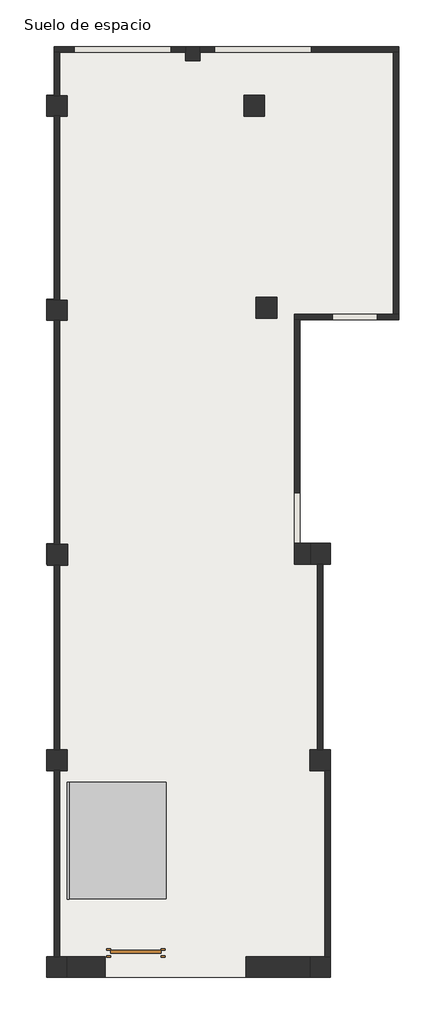
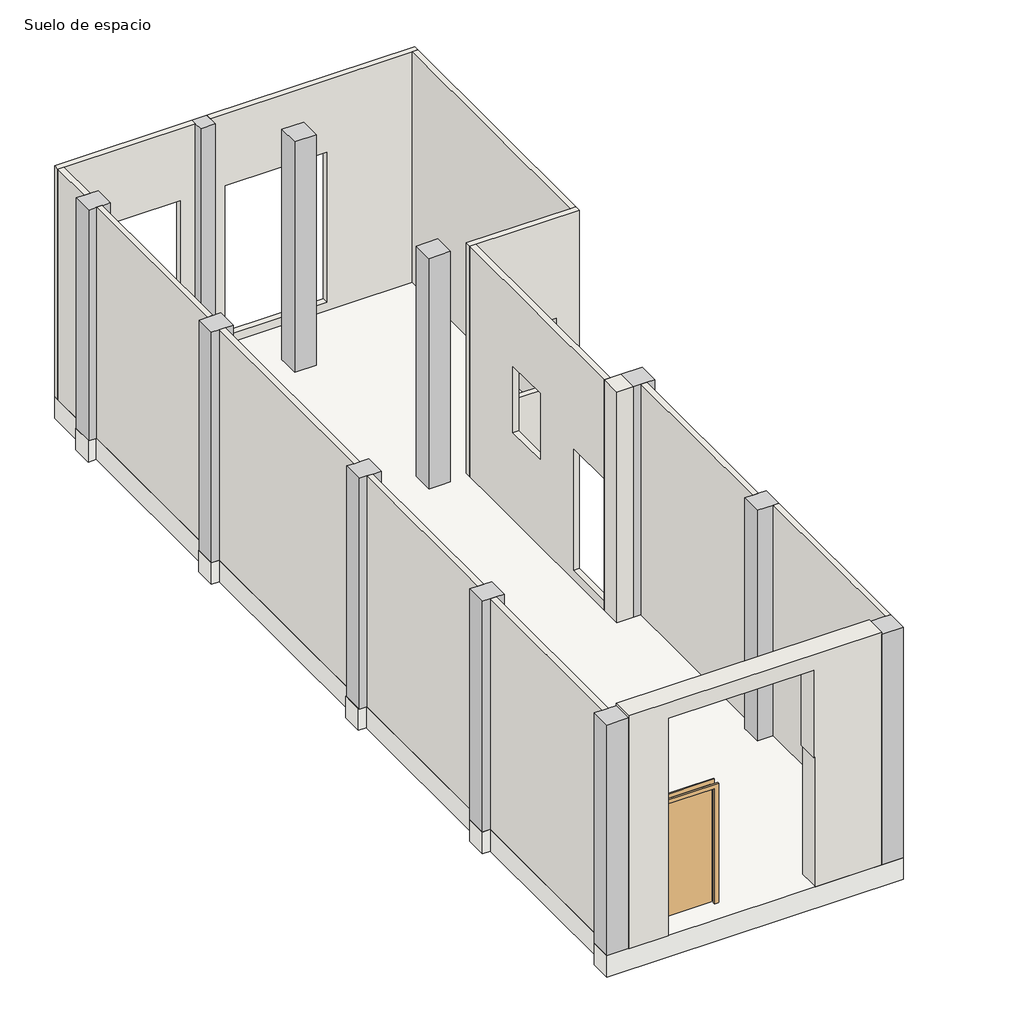
# One storey: 14 walls, 11 columns, 1 door, 1 railing, 1 ramp, 1 slab.
"""IFC4 building model written with IfcOpenShell, lengths in millimetres."""

import ifcopenshell
import ifcopenshell.guid

model = None  # the IFC model being written
_history = None  # IfcOwnerHistory: only IFC2X3 demands one
_inside = {}  # id of a spatial element -> (the spatial element, [elements in it])
_under = {}  # id of a project, library or spatial element -> (it, [spatial elements below it])
_declared = {}  # id of a project -> (the project, [libraries it declares])
_typed = {}  # id of a type object -> (the type object, [elements of that type])
_made_of = {}  # id of a material, layer set ... -> (it, [elements and type objects made of it])


def new_model(schema):
    """Start an empty IFC model of exactly this schema.

    Asked for "IFC4X3", IfcOpenShell would pick the latest addendum, in which some entities
    have other attributes; the version numbers below select the first issue.
    IFC2X3 requires an IfcOwnerHistory on every rooted entity: one is made here for all.
    """
    global model, _history
    if schema == "IFC4X3":
        model = ifcopenshell.file(schema_version=(4, 3, 0, 0))
    else:
        model = ifcopenshell.file(schema=schema)
    _inside.clear()
    _under.clear()
    _declared.clear()
    _typed.clear()
    _made_of.clear()
    _history = None
    if model.schema == "IFC2X3":
        org = make("IfcOrganization", Name="unknown")
        user = make(
            "IfcPersonAndOrganization",
            ThePerson=make("IfcPerson", FamilyName="unknown"),
            TheOrganization=org,
        )
        app = make(
            "IfcApplication",
            ApplicationDeveloper=org,
            Version="unknown",
            ApplicationFullName="unknown",
            ApplicationIdentifier="unknown",
        )
        _history = make(
            "IfcOwnerHistory",
            OwningUser=user,
            OwningApplication=app,
            ChangeAction="ADDED",
            CreationDate=0,
        )
    return model


def make(cls, **values):
    """One entity of the class cls with the attributes given. An attribute that is None is left unset."""
    return model.create_entity(
        cls, **{name: value for name, value in values.items() if value is not None}
    )


def rooted(cls, **values):
    """An entity with a GlobalId (a new one), such as an element, a storey or a relation."""
    return make(cls, GlobalId=ifcopenshell.guid.new(), OwnerHistory=_history, **values)


def si_unit(unit_type, name, prefix=None):
    """IfcSIUnit, for example si_unit("LENGTHUNIT", "METRE", prefix="MILLI")."""
    return make("IfcSIUnit", UnitType=unit_type, Prefix=prefix, Name=name)


def assignment(units):
    """IfcUnitAssignment: the units of a project."""
    return None if units is None else make("IfcUnitAssignment", Units=units)


def point(xyz):
    """IfcCartesianPoint."""
    return None if xyz is None else make("IfcCartesianPoint", Coordinates=xyz)


def direction(xyz):
    """IfcDirection."""
    return None if xyz is None else make("IfcDirection", DirectionRatios=xyz)


def frame(location, z_axis=None, x_axis=None):
    """IfcAxis2Placement3D, a coordinate frame: its origin and axes. An axis left out is left unset."""
    return make(
        "IfcAxis2Placement3D",
        Location=point(location),
        Axis=direction(z_axis),
        RefDirection=direction(x_axis),
    )


def origin():
    """The frame at (0, 0, 0) with its axes left unset."""
    return frame((0.0, 0.0, 0.0))


def origin_with_axes():
    """The frame at (0, 0, 0) with the z axis (0, 0, 1) and the x axis (1, 0, 0) written out."""
    return frame((0.0, 0.0, 0.0), z_axis=(0.0, 0.0, 1.0), x_axis=(1.0, 0.0, 0.0))


def place(relative_to, where):
    """IfcLocalPlacement: puts the frame where relative to a parent placement (None: the world)."""
    return make(
        "IfcLocalPlacement", PlacementRelTo=relative_to, RelativePlacement=where
    )


def context(
    kind, dimensions, precision=None, world=None, true_north=None, identifier=None
):
    """IfcGeometricRepresentationContext, for example the 3D "Model" context."""
    return make(
        "IfcGeometricRepresentationContext",
        ContextIdentifier=identifier,
        ContextType=kind,
        CoordinateSpaceDimension=dimensions,
        Precision=precision,
        WorldCoordinateSystem=world,
        TrueNorth=true_north,
    )


def project(units=None, contexts=None):
    """IfcProject with its units and contexts."""
    return rooted(
        "IfcProject",
        Name="project",
        RepresentationContexts=contexts,
        UnitsInContext=assignment(units),
    )


def spatial(cls, under=None, at=None, **own):
    """A site, building, storey or space (cls), placed at a placement, below another one or the project."""
    s = rooted(cls, ObjectPlacement=at, **own)
    if under is not None:
        _under.setdefault(under.id(), (under, []))[1].append(s)
    return s


def polyline(points):
    """IfcPolyline through the points."""
    return make("IfcPolyline", Points=[point(p) for p in points])


def ellipse_curve(where, semi_axis1, semi_axis2):
    """IfcEllipse in the frame where."""
    return make(
        "IfcEllipse", Position=where, SemiAxis1=semi_axis1, SemiAxis2=semi_axis2
    )


def outline(outer, holes=None, kind="AREA"):
    """IfcArbitraryClosedProfileDef: a profile drawn as a closed curve; with holes, ...WithVoids."""
    if holes is None:
        return make("IfcArbitraryClosedProfileDef", ProfileType=kind, OuterCurve=outer)
    return make(
        "IfcArbitraryProfileDefWithVoids",
        ProfileType=kind,
        OuterCurve=outer,
        InnerCurves=holes,
    )


def extrude(swept, where, along, depth):
    """IfcExtrudedAreaSolid: the profile swept, set in the frame where, extruded along a direction by depth."""
    return make(
        "IfcExtrudedAreaSolid",
        SweptArea=swept,
        Position=where,
        ExtrudedDirection=direction(along),
        Depth=depth,
    )


def faces_of(points, faces, orient=None, outer=None):
    """IfcFace entities. A face is a list of loops; a loop is a list of indices into points, from 0.

    orient and outer hold one flag for each loop. By default every Orientation is true, the
    first loop of a face is its IfcFaceOuterBound and the others are IfcFaceBound.
    """
    made = []
    for i, loops in enumerate(faces):
        bounds = []
        for j, loop in enumerate(loops):
            is_outer = j == 0 if outer is None else outer[i][j]
            bounds.append(
                make(
                    "IfcFaceOuterBound" if is_outer else "IfcFaceBound",
                    Bound=make("IfcPolyLoop", Polygon=[points[k] for k in loop]),
                    Orientation=True if orient is None else orient[i][j],
                )
            )
        made.append(make("IfcFace", Bounds=bounds))
    return made


def faceted_brep(points, faces, orient=None, outer=None, voids=None):
    """IfcFacetedBrep: a solid bounded by flat faces; with voids (closed shells), ...WithVoids."""
    shared = [point(p) for p in points]
    hull = make("IfcClosedShell", CfsFaces=faces_of(shared, faces, orient, outer))
    if voids is None:
        return make("IfcFacetedBrep", Outer=hull)
    return make(
        "IfcFacetedBrepWithVoids",
        Outer=hull,
        Voids=[
            make(cls, CfsFaces=faces_of(shared, fs, o, b)) for cls, fs, o, b in voids
        ],
    )


def shape(context_of_items, identifier, shape_type, items):
    """IfcShapeRepresentation: the items that make up one representation, for example the "Body"."""
    return make(
        "IfcShapeRepresentation",
        ContextOfItems=context_of_items,
        RepresentationIdentifier=identifier,
        RepresentationType=shape_type,
        Items=items,
    )


def source(mapping_origin, context_of_items, identifier, shape_type, items):
    """IfcRepresentationMap: a shape defined once, which mapped items show again and again."""
    return make(
        "IfcRepresentationMap",
        MappingOrigin=mapping_origin,
        MappedRepresentation=shape(context_of_items, identifier, shape_type, items),
    )


def transform(
    local_origin,
    x_axis=None,
    y_axis=None,
    z_axis=None,
    scale=None,
    scale2=None,
    scale3=None,
    uniform=True,
):
    """IfcCartesianTransformationOperator3D, or its non-uniform kind. x_axis, y_axis, z_axis: its Axis1, 2, 3."""
    if uniform:
        return make(
            "IfcCartesianTransformationOperator3D",
            Axis1=direction(x_axis),
            Axis2=direction(y_axis),
            LocalOrigin=point(local_origin),
            Scale=scale,
            Axis3=direction(z_axis),
        )
    return make(
        "IfcCartesianTransformationOperator3DnonUniform",
        Axis1=direction(x_axis),
        Axis2=direction(y_axis),
        LocalOrigin=point(local_origin),
        Scale=scale,
        Axis3=direction(z_axis),
        Scale2=scale2,
        Scale3=scale3,
    )


def mapped(mapping_source, mapping_target):
    """IfcMappedItem: shows the shape of a source again, moved by a transform."""
    return make(
        "IfcMappedItem", MappingSource=mapping_source, MappingTarget=mapping_target
    )


def made_of(thing, what):
    """Note that an element or type object is made of a material, layer set ...; save() writes the relation."""
    if what is not None:
        _made_of.setdefault(what.id(), (what, []))[1].append(thing)
    return thing


def element(
    cls,
    number,
    at=None,
    inside=None,
    cuts=None,
    type_object=None,
    material=None,
    context=None,
    identifier="Body",
    shape_type=None,
    held_by="IfcProductDefinitionShape",
    body=None,
    shapes=None,
    **own,
):
    """One element of the class cls, such as IfcWall. Its Tag is "e" and its number.

    at: its placement. inside: the storey or other place that contains it. cuts: it is an
    opening in that element (IfcRelVoidsElement). A single representation is given by context,
    identifier, shape_type and body (its items); several are given by shapes. held_by: the class
    of the entity that holds the representations. save() writes the other relations.
    """
    e = rooted(cls, Tag="e%d" % number, ObjectPlacement=at, **own)
    if body is not None:
        shapes = [shape(context, identifier, shape_type, body)]
    if shapes is not None:
        e.Representation = make(held_by, Representations=shapes)
    if inside is not None:
        _inside.setdefault(inside.id(), (inside, []))[1].append(e)
    if cuts is not None:
        rooted(
            "IfcRelVoidsElement", RelatingBuildingElement=cuts, RelatedOpeningElement=e
        )
    if type_object is not None:
        _typed.setdefault(type_object.id(), (type_object, []))[1].append(e)
    return made_of(e, material)


def aggregate(whole, parts):
    """IfcRelAggregates: a whole, such as a stair, and the parts it consists of."""
    return rooted("IfcRelAggregates", RelatingObject=whole, RelatedObjects=parts)


def save(model, path):
    """Write the relations noted so far, then the file.

    IfcRelAggregates (storeys below a building ...), IfcRelContainedInSpatialStructure (elements
    in a storey), IfcRelDefinesByType, IfcRelAssociatesMaterial and IfcRelDeclares: one each for
    every whole, place, type object, material and project.
    """
    for whole, parts in _under.values():
        aggregate(whole, parts)
    for where, things in _inside.values():
        rooted(
            "IfcRelContainedInSpatialStructure",
            RelatedElements=things,
            RelatingStructure=where,
        )
    for kind, things in _typed.values():
        rooted("IfcRelDefinesByType", RelatedObjects=things, RelatingType=kind)
    for what, things in _made_of.values():
        rooted("IfcRelAssociatesMaterial", RelatedObjects=things, RelatingMaterial=what)
    for by, libraries in _declared.values():
        rooted("IfcRelDeclares", RelatingContext=by, RelatedDefinitions=libraries)
    model.write(path)


def plane_surface(at):
    """IfcPlane: the flat surface through the origin of the frame at, square to its z axis."""
    return make("IfcPlane", Position=at)


def cylinder_surface(at, radius):
    """IfcCylindricalSurface: all points at the distance radius from the z axis of the frame at."""
    return make("IfcCylindricalSurface", Position=at, Radius=radius)


def advanced_brep(points, edges, surfaces, faces):
    """IfcAdvancedBrep: a solid bounded by faces that lie on surfaces and meet in shared edges.

    An edge is (start, end): straight between two places in points (the first is 0);
    or (start, end, curve); or (start, end, curve, False) where it runs against its curve.
    A face is (place in surfaces, loops), or (place, loops, False) where it looks against
    its surface's normal. A loop lists edges by number (the first is 1), with a minus sign
    where the edge is run from its end to its start. The first loop is the outer one.
    """
    corners = [point(p) for p in points]
    vertices = [make("IfcVertexPoint", VertexGeometry=c) for c in corners]
    made = []
    for start, end, *more in edges:
        made.append(
            make(
                "IfcEdgeCurve",
                EdgeStart=vertices[start],
                EdgeEnd=vertices[end],
                EdgeGeometry=more[0] if more else make("IfcPolyline", Points=[corners[start], corners[end]]),
                SameSense=more[1] if len(more) > 1 else True,
            )
        )
    hull = []
    for where, loops, *sense in faces:
        bounds = []
        for j, loop in enumerate(loops):
            ring = [make("IfcOrientedEdge", EdgeElement=made[abs(k) - 1], Orientation=k > 0) for k in loop]
            bounds.append(
                make(
                    "IfcFaceOuterBound" if j == 0 else "IfcFaceBound",
                    Bound=make("IfcEdgeLoop", EdgeList=ring),
                    Orientation=True,
                )
            )
        hull.append(make("IfcAdvancedFace", Bounds=bounds, FaceSurface=surfaces[where], SameSense=sense[0] if sense else True))
    return make("IfcAdvancedBrep", Outer=make("IfcClosedShell", CfsFaces=hull))


def m_rectangular_column_380_x_380mm_f7aa0fc7(model_context):
    return source(origin(), model_context, "Body", "SweptSolid", [
        extrude(outline(polyline([(190.0, 190.0), (190.0, -190.0), (-190.0, -190.0), (-190.0, 190.0), (190.0, 190.0)])), frame((0.0, 0.0, 40.0), z_axis=(0.0, 0.0, 1.0), x_axis=(1.0, 0.0, 0.0)), (0.0, 0.0, 1.0), 4260.0),
    ])


def m_single_flush_0915_x_2134mm_17617764(model_context):
    return source(origin(), model_context, "Body", "SweptSolid", [
        extrude(outline(polyline([(2210.0, -533.5), (0.0, -533.5), (0.0, -457.5), (2134.0, -457.5), (2134.0, 457.5), (0.0, 457.5), (0.0, 533.5), (2210.0, 533.5), (2210.0, -533.5)])), frame((0.0, -75.0, 0.0), z_axis=(0.0, 1.0, 0.0), x_axis=(0.0, 0.0, 1.0)), (0.0, 0.0, 1.0), 25.0),
        extrude(outline(polyline([(2210.0, 533.5), (2210.0, -533.5), (0.0, -533.5), (0.0, -457.5), (2134.0, -457.5), (2134.0, 457.5), (0.0, 457.5), (0.0, 533.5), (2210.0, 533.5)])), frame((0.0, 50.0, 0.0), z_axis=(0.0, 1.0, 0.0), x_axis=(0.0, 0.0, 1.0)), (0.0, 0.0, 1.0), 25.0),
        extrude(outline(polyline([(457.5, 1.0), (457.5, -50.0), (-457.5, -50.0), (-457.5, 1.0), (457.5, 1.0)])), origin_with_axes(), (0.0, 0.0, 1.0), 2134.0),
    ])


def ramp_1_b614bedc(model_context):
    return source(origin(), model_context, "Body", "SweptSolid", [
        extrude(outline(polyline([(-588.7354398, 40.0), (1550.939444, 200.0), (1550.939444, 49.5812066), (-588.7354398, -110.4187934), (-588.7354398, 40.0)])), frame((5737.3508412, 0.0, 0.0), z_axis=(1.0, 0.0, 0.0), x_axis=(0.0, 1.0, 0.0)), (0.0, 0.0, 1.0), 1790.0),
    ])


model = new_model("IFC4")

# Units and contexts
model_context = context("Model", 3, world=origin())
ifc_project = project(units=[si_unit("LENGTHUNIT", "METRE", prefix="MILLI")], contexts=[model_context])

# Site, building, storey
site = spatial("IfcSite", under=ifc_project)
building = spatial("IfcBuilding", under=site)
storey = spatial("IfcBuildingStorey", under=building, Name="Suelo de espacio", Elevation=40.0)

# Columns
placement = place(None, origin())
element("IfcColumn", 1, ObjectType="M_Rectangular Column : 260 x 260mm", at=placement, inside=storey, context=model_context, shape_type="Brep", body=[
    faceted_brep([(8142.3508412, 14950.939444, 4300.0), (7882.3508412, 14950.939444, 4300.0), (7882.3508412, 14850.939444, 4300.0), (7882.3508412, 14690.939444, 4300.0), (8142.3508412, 14690.939444, 4300.0), (8142.3508412, 14850.939444, 4300.0), (8142.3508412, 14950.939444, 40.0), (8142.3508412, 14850.939444, 40.0), (8142.3508412, 14690.939444, 40.0), (7882.3508412, 14690.939444, 40.0), (7882.3508412, 14850.939444, 40.0), (7882.3508412, 14950.939444, 40.0)], [[[0, 1, 2, 3, 4, 5]], [[6, 7, 8, 9, 10, 11]], [[1, 0, 6, 11]], [[3, 2, 1, 11, 10, 9]], [[4, 3, 9, 8]], [[0, 5, 4, 8, 7, 6]]]),
])
element("IfcColumn", 2, ObjectType="M_Rectangular Column : 380 x 370mm", at=placement, inside=storey, context=model_context, shape_type="Brep", body=[
    faceted_brep([(5722.3508412, 10330.939444, 4300.0), (5342.3508412, 10330.939444, 4300.0), (5342.3508412, 9960.939444, 4300.0), (5482.3508412, 9960.939444, 4300.0), (5582.3508412, 9960.939444, 4300.0), (5722.3508412, 9960.939444, 4300.0), (5722.3508412, 10330.939444, 40.0), (5722.3508412, 9960.939444, 40.0), (5582.3508412, 9960.939444, 40.0), (5482.3508412, 9960.939444, 40.0), (5342.3508412, 9960.939444, 40.0), (5342.3508412, 10330.939444, 40.0)], [[[0, 1, 2, 3, 4, 5]], [[6, 7, 8, 9, 10, 11]], [[1, 0, 6, 11]], [[2, 1, 11, 10]], [[5, 4, 3, 2, 10, 9, 8, 7]], [[0, 5, 7, 6]]]),
])
element("IfcColumn", 3, ObjectType="M_Rectangular Column : 380 x 370mm", at=placement, inside=storey, context=model_context, shape_type="Brep", body=[
    faceted_brep([(5722.3508412, 14050.939444, 4300.0), (5582.3508412, 14050.939444, 4300.0), (5482.3508412, 14050.939444, 4300.0), (5342.3508412, 14050.939444, 4300.0), (5342.3508412, 13680.939444, 4300.0), (5482.3508412, 13680.939444, 4300.0), (5482.3508412, 13685.939444, 4300.0), (5582.3508412, 13685.939444, 4300.0), (5582.3508412, 13680.939444, 4300.0), (5722.3508412, 13680.939444, 4300.0), (5722.3508412, 14050.939444, 40.0), (5722.3508412, 13680.939444, 40.0), (5582.3508412, 13680.939444, 40.0), (5582.3508412, 13685.939444, 40.0), (5482.3508412, 13685.939444, 40.0), (5482.3508412, 13680.939444, 40.0), (5342.3508412, 13680.939444, 40.0), (5342.3508412, 14050.939444, 40.0), (5482.3508412, 14050.939444, 40.0), (5582.3508412, 14050.939444, 40.0)], [[[0, 1, 2, 3, 4, 5, 6, 7, 8, 9]], [[10, 11, 12, 13, 14, 15, 16, 17, 18, 19]], [[3, 2, 1, 0, 10, 19, 18, 17]], [[4, 3, 17, 16]], [[4, 16, 15, 5]], [[0, 9, 11, 10]], [[7, 13, 12, 8]], [[14, 6, 5, 15]], [[13, 7, 6, 14]], [[11, 9, 8, 12]]]),
])
element("IfcColumn", 4, ObjectType="M_Rectangular Column : 380 x 380mm", at=placement, inside=storey, context=model_context, shape_type="Brep", body=[
    faceted_brep([(5722.3508412, -1629.060556, 4300.0), (5582.3508412, -1629.060556, 4300.0), (5482.3508412, -1629.060556, 4300.0), (5342.3508412, -1629.060556, 4300.0), (5342.3508412, -2009.060556, 4300.0), (5722.3508412, -2009.060556, 4300.0), (5722.3508412, -1629.060556, 40.0), (5722.3508412, -2009.060556, 40.0), (5342.3508412, -2009.060556, 40.0), (5342.3508412, -1629.060556, 40.0), (5482.3508412, -1629.060556, 40.0), (5582.3508412, -1629.060556, 40.0)], [[[0, 1, 2, 3, 4, 5]], [[6, 7, 8, 9, 10, 11]], [[3, 2, 1, 0, 6, 11, 10, 9]], [[4, 3, 9, 8]], [[5, 4, 8, 7]], [[0, 5, 7, 6]]]),
])
element("IfcColumn", 5, ObjectType="M_Rectangular Column : 380 x 380mm", at=placement, inside=storey, context=model_context, shape_type="Brep", body=[
    faceted_brep([(10522.3508412, -1629.060556, 4300.0), (10422.3508412, -1629.060556, 4300.0), (10142.3508412, -1629.060556, 4300.0), (10142.3508412, -2009.060556, 4300.0), (10522.3508412, -2009.060556, 4300.0), (10522.3508412, -1629.060556, 40.0), (10522.3508412, -2009.060556, 40.0), (10142.3508412, -2009.060556, 40.0), (10142.3508412, -1629.060556, 40.0), (10422.3508412, -1629.060556, 40.0)], [[[0, 1, 2, 3, 4]], [[5, 6, 7, 8, 9]], [[2, 1, 0, 5, 9, 8]], [[3, 2, 8, 7]], [[4, 3, 7, 6]], [[0, 4, 6, 5]]]),
])
element("IfcColumn", 6, ObjectType="M_Rectangular Column : 380 x 380mm", at=placement, inside=storey, context=model_context, shape_type="Brep", body=[
    faceted_brep([(5722.3508412, 2140.939444, 4300.0), (5582.3508412, 2140.939444, 4300.0), (5482.3508412, 2140.939444, 4300.0), (5342.3508412, 2140.939444, 4300.0), (5342.3508412, 1760.939444, 4300.0), (5482.3508412, 1760.939444, 4300.0), (5482.3508412, 1761.3849652, 4300.0), (5582.3508412, 1761.3849652, 4300.0), (5582.3508412, 1760.939444, 4300.0), (5722.3508412, 1760.939444, 4300.0), (5722.3508412, 2140.939444, 40.0), (5722.3508412, 1760.939444, 40.0), (5582.3508412, 1760.939444, 40.0), (5582.3508412, 1761.3849652, 40.0), (5482.3508412, 1761.3849652, 40.0), (5482.3508412, 1760.939444, 40.0), (5342.3508412, 1760.939444, 40.0), (5342.3508412, 2140.939444, 40.0), (5482.3508412, 2140.939444, 40.0), (5582.3508412, 2140.939444, 40.0)], [[[0, 1, 2, 3, 4, 5, 6, 7, 8, 9]], [[10, 11, 12, 13, 14, 15, 16, 17, 18, 19]], [[3, 2, 1, 0, 10, 19, 18, 17]], [[4, 3, 17, 16]], [[4, 16, 15, 5]], [[0, 9, 11, 10]], [[7, 13, 12, 8]], [[14, 6, 5, 15]], [[11, 9, 8, 12]], [[13, 7, 6, 14]]]),
])
element("IfcColumn", 7, ObjectType="M_Rectangular Column : 380 x 380mm", at=placement, inside=storey, context=model_context, shape_type="Brep", body=[
    faceted_brep([(10522.3508412, 2140.939444, 4300.0), (10382.3508412, 2140.939444, 4300.0), (10282.3508412, 2140.939444, 4300.0), (10142.3508412, 2140.939444, 4300.0), (10142.3508412, 1760.939444, 4300.0), (10422.3508412, 1760.939444, 4300.0), (10522.3508412, 1760.939444, 4300.0), (10522.3508412, 2140.939444, 40.0), (10522.3508412, 1760.939444, 40.0), (10422.3508412, 1760.939444, 40.0), (10142.3508412, 1760.939444, 40.0), (10142.3508412, 2140.939444, 40.0), (10282.3508412, 2140.939444, 40.0), (10382.3508412, 2140.939444, 40.0)], [[[0, 1, 2, 3, 4, 5, 6]], [[7, 8, 9, 10, 11, 12, 13]], [[3, 2, 1, 0, 7, 13, 12, 11]], [[4, 3, 11, 10]], [[6, 5, 4, 10, 9, 8]], [[0, 6, 8, 7]]]),
])
element("IfcColumn", 8, ObjectType="M_Rectangular Column : 380 x 380mm", at=placement, inside=storey, context=model_context, shape_type="Brep", body=[
    faceted_brep([(5732.3508412, 5880.939444, 4300.0), (5582.3508412, 5880.939444, 4300.0), (5482.3508412, 5880.939444, 4300.0), (5352.3508412, 5880.939444, 4300.0), (5352.3508412, 5500.939444, 4300.0), (5482.3508412, 5500.939444, 4300.0), (5582.3508412, 5500.939444, 4300.0), (5732.3508412, 5500.939444, 4300.0), (5732.3508412, 5880.939444, 40.0), (5732.3508412, 5500.939444, 40.0), (5582.3508412, 5500.939444, 40.0), (5482.3508412, 5500.939444, 40.0), (5352.3508412, 5500.939444, 40.0), (5352.3508412, 5880.939444, 40.0), (5482.3508412, 5880.939444, 40.0), (5582.3508412, 5880.939444, 40.0)], [[[0, 1, 2, 3, 4, 5, 6, 7]], [[8, 9, 10, 11, 12, 13, 14, 15]], [[3, 2, 1, 0, 8, 15, 14, 13]], [[4, 3, 13, 12]], [[7, 6, 5, 4, 12, 11, 10, 9]], [[0, 7, 9, 8]]]),
])
element("IfcColumn", 9, ObjectType="M_Rectangular Column : 380 x 380mm", at=placement, inside=storey, context=model_context, shape_type="Brep", body=[
    faceted_brep([(10522.3508412, 5520.939444, 4300.0), (10522.3508412, 5900.939444, 4300.0), (10152.3508412, 5900.939444, 4300.0), (10152.3508412, 5520.939444, 4300.0), (10282.3508412, 5520.939444, 4300.0), (10382.3508412, 5520.939444, 4300.0), (10522.3508412, 5900.939444, 40.0), (10522.3508412, 5520.939444, 40.0), (10382.3508412, 5520.939444, 40.0), (10282.3508412, 5520.939444, 40.0), (10152.3508412, 5520.939444, 40.0), (10152.3508412, 5900.939444, 40.0)], [[[0, 1, 2, 3, 4, 5]], [[6, 7, 8, 9, 10, 11]], [[1, 6, 11, 2]], [[7, 0, 5, 4, 3, 10, 9, 8]], [[1, 0, 7, 6]], [[3, 2, 11, 10]]]),
])
m_rectangular_column_380_x_380mm_shape = m_rectangular_column_380_x_380mm_f7aa0fc7(model_context)
element("IfcColumn", 10, ObjectType="M_Rectangular Column : 380 x 380mm", at=placement, inside=storey, context=model_context, shape_type="MappedRepresentation", body=[
    mapped(m_rectangular_column_380_x_380mm_shape, transform((9132.3508412, 13870.939444, 0.0), x_axis=(1.0, 0.0, 0.0), y_axis=(0.0, 1.0, 0.0), z_axis=(0.0, 0.0, 1.0))),
])
element("IfcColumn", 11, ObjectType="M_Rectangular Column : 380 x 380mm", at=placement, inside=storey, context=model_context, shape_type="MappedRepresentation", body=[
    mapped(m_rectangular_column_380_x_380mm_shape, transform((9352.3508412, 10190.939444, 0.0), x_axis=(1.0, 0.0, 0.0), y_axis=(0.0, 1.0, 0.0), z_axis=(0.0, 0.0, 1.0))),
])

# Door
m_single_flush_0915_x_2134mm_shape = m_single_flush_0915_x_2134mm_17617764(model_context)
element("IfcDoor", 12, ObjectType="M_Single-Flush : 0915 x 2134mm", at=placement, inside=storey, context=model_context, shape_type="MappedRepresentation", body=[
    mapped(m_single_flush_0915_x_2134mm_shape, transform((6972.3508412, -1564.060556, 40.0), x_axis=(-1.0, 0.0, 0.0), y_axis=(0.0, -1.0, 0.0), z_axis=(0.0, 0.0, 1.0))),
])

# Railing
element("IfcRailing", 13, ObjectType="900mm Pipe", at=placement, inside=storey, context=model_context, shape_type="AdvancedBrep", body=[
    advanced_brep(
    [(5757.3508412, -588.7354398, 919.9441609), (5717.3508412, -588.7354398, 919.9441609), (5757.3508412, 1550.939444, 1079.9441609), (5717.3508412, 1550.939444, 1079.9441609)],
    [
        (0, 1, ellipse_curve(frame((5737.3508412, -588.7354398, 919.9441609), z_axis=(0.0, -1.0, 0.0), x_axis=(0.0, 0.0, -1.0)), 20.0558391, 20.0)),
        (1, 0, ellipse_curve(frame((5737.3508412, -588.7354398, 919.9441609), z_axis=(0.0, -1.0, 0.0), x_axis=(0.0, 0.0, -1.0)), 20.0558391, 20.0)),
        (2, 3, ellipse_curve(frame((5737.3508412, 1550.939444, 1079.9441609), z_axis=(0.0, 1.0, 0.0), x_axis=(0.0, 0.0, -1.0)), 20.0558391, 20.0)),
        (3, 2, ellipse_curve(frame((5737.3508412, 1550.939444, 1079.9441609), z_axis=(0.0, 1.0, 0.0), x_axis=(0.0, 0.0, -1.0)), 20.0558391, 20.0)),
        (0, 2),
        (3, 1),
    ],
    [
        plane_surface(frame((5737.3508412, -588.7354398, 940.0), z_axis=(0.0, -1.0, 0.0), x_axis=(0.0, 0.0, 1.0))),
        plane_surface(frame((5737.3508412, 1550.939444, 1100.0), z_axis=(0.0, 1.0, 0.0), x_axis=(0.0, 0.0, 1.0))),
        cylinder_surface(frame((5737.3508412, -587.2440494, 920.0556837), z_axis=(0.0, -0.9972158174462339, -0.07456952081809044), x_axis=(-1.0, 0.0, 0.0)), 20.0),
    ],
    [
        (0, [[1, 2]]),
        (1, [[3, 4]]),
        (2, [[-1, 5, -4, 6]]),
        (2, [[-2, -6, -3, -5]]),
    ],
),
    advanced_brep(
    [(5722.3508412, -588.7354398, 799.9581207), (5752.3508412, -588.7354398, 799.9581207), (5722.3508412, 1550.939444, 959.9581207), (5752.3508412, 1550.939444, 959.9581207)],
    [
        (0, 1, ellipse_curve(frame((5737.3508412, -588.7354398, 799.9581207), z_axis=(0.0, -1.0, 0.0), x_axis=(0.0, 0.0, -1.0)), 15.0418793, 15.0)),
        (1, 0, ellipse_curve(frame((5737.3508412, -588.7354398, 799.9581207), z_axis=(0.0, -1.0, 0.0), x_axis=(0.0, 0.0, -1.0)), 15.0418793, 15.0)),
        (2, 3, ellipse_curve(frame((5737.3508412, 1550.939444, 959.9581207), z_axis=(0.0, 1.0, 0.0), x_axis=(0.0, 0.0, -1.0)), 15.0418793, 15.0)),
        (3, 2, ellipse_curve(frame((5737.3508412, 1550.939444, 959.9581207), z_axis=(0.0, 1.0, 0.0), x_axis=(0.0, 0.0, -1.0)), 15.0418793, 15.0)),
        (0, 2),
        (3, 1),
    ],
    [
        plane_surface(frame((5737.3508412, -588.7354398, 815.0), z_axis=(0.0, -1.0, 0.0), x_axis=(0.0, 0.0, 1.0))),
        plane_surface(frame((5737.3508412, 1550.939444, 975.0), z_axis=(0.0, 1.0, 0.0), x_axis=(0.0, 0.0, 1.0))),
        cylinder_surface(frame((5737.3508412, -587.616897, 800.0417627), z_axis=(0.0, -0.9972158174462339, -0.07456952081809044), x_axis=(1.0, 0.0, 0.0)), 15.0),
    ],
    [
        (0, [[1, 2]]),
        (1, [[3, 4]]),
        (2, [[-1, 5, -4, 6]]),
        (2, [[-2, -6, -3, -5]]),
    ],
),
    advanced_brep(
    [(5722.3508412, -588.7354398, 674.9581207), (5752.3508412, -588.7354398, 674.9581207), (5722.3508412, 1550.939444, 834.9581207), (5752.3508412, 1550.939444, 834.9581207)],
    [
        (0, 1, ellipse_curve(frame((5737.3508412, -588.7354398, 674.9581207), z_axis=(0.0, -1.0, 0.0), x_axis=(0.0, 0.0, -1.0)), 15.0418793, 15.0)),
        (1, 0, ellipse_curve(frame((5737.3508412, -588.7354398, 674.9581207), z_axis=(0.0, -1.0, 0.0), x_axis=(0.0, 0.0, -1.0)), 15.0418793, 15.0)),
        (2, 3, ellipse_curve(frame((5737.3508412, 1550.939444, 834.9581207), z_axis=(0.0, 1.0, 0.0), x_axis=(0.0, 0.0, -1.0)), 15.0418793, 15.0)),
        (3, 2, ellipse_curve(frame((5737.3508412, 1550.939444, 834.9581207), z_axis=(0.0, 1.0, 0.0), x_axis=(0.0, 0.0, -1.0)), 15.0418793, 15.0)),
        (0, 2),
        (3, 1),
    ],
    [
        plane_surface(frame((5737.3508412, -588.7354398, 690.0), z_axis=(0.0, -1.0, 0.0), x_axis=(0.0, 0.0, 1.0))),
        plane_surface(frame((5737.3508412, 1550.939444, 850.0), z_axis=(0.0, 1.0, 0.0), x_axis=(0.0, 0.0, 1.0))),
        cylinder_surface(frame((5737.3508412, -587.616897, 675.0417627), z_axis=(0.0, -0.9972158174462339, -0.07456952081809044), x_axis=(1.0, 0.0, 0.0)), 15.0),
    ],
    [
        (0, [[1, 2]]),
        (1, [[3, 4]]),
        (2, [[-1, 5, -4, 6]]),
        (2, [[-2, -6, -3, -5]]),
    ],
),
    advanced_brep(
    [(5722.3508412, -588.7354398, 549.9581207), (5752.3508412, -588.7354398, 549.9581207), (5722.3508412, 1550.939444, 709.9581207), (5752.3508412, 1550.939444, 709.9581207)],
    [
        (0, 1, ellipse_curve(frame((5737.3508412, -588.7354398, 549.9581207), z_axis=(0.0, -1.0, 0.0), x_axis=(0.0, 0.0, -1.0)), 15.0418793, 15.0)),
        (1, 0, ellipse_curve(frame((5737.3508412, -588.7354398, 549.9581207), z_axis=(0.0, -1.0, 0.0), x_axis=(0.0, 0.0, -1.0)), 15.0418793, 15.0)),
        (2, 3, ellipse_curve(frame((5737.3508412, 1550.939444, 709.9581207), z_axis=(0.0, 1.0, 0.0), x_axis=(0.0, 0.0, -1.0)), 15.0418793, 15.0)),
        (3, 2, ellipse_curve(frame((5737.3508412, 1550.939444, 709.9581207), z_axis=(0.0, 1.0, 0.0), x_axis=(0.0, 0.0, -1.0)), 15.0418793, 15.0)),
        (0, 2),
        (3, 1),
    ],
    [
        plane_surface(frame((5737.3508412, -588.7354398, 565.0), z_axis=(0.0, -1.0, 0.0), x_axis=(0.0, 0.0, 1.0))),
        plane_surface(frame((5737.3508412, 1550.939444, 725.0), z_axis=(0.0, 1.0, 0.0), x_axis=(0.0, 0.0, 1.0))),
        cylinder_surface(frame((5737.3508412, -587.616897, 550.0417627), z_axis=(0.0, -0.9972158174462339, -0.07456952081809044), x_axis=(1.0, 0.0, 0.0)), 15.0),
    ],
    [
        (0, [[1, 2]]),
        (1, [[3, 4]]),
        (2, [[-1, 5, -4, 6]]),
        (2, [[-2, -6, -3, -5]]),
    ],
),
    advanced_brep(
    [(5722.3508412, -588.7354398, 424.9581207), (5752.3508412, -588.7354398, 424.9581207), (5722.3508412, 1550.939444, 584.9581207), (5752.3508412, 1550.939444, 584.9581207)],
    [
        (0, 1, ellipse_curve(frame((5737.3508412, -588.7354398, 424.9581207), z_axis=(0.0, -1.0, 0.0), x_axis=(0.0, 0.0, -1.0)), 15.0418793, 15.0)),
        (1, 0, ellipse_curve(frame((5737.3508412, -588.7354398, 424.9581207), z_axis=(0.0, -1.0, 0.0), x_axis=(0.0, 0.0, -1.0)), 15.0418793, 15.0)),
        (2, 3, ellipse_curve(frame((5737.3508412, 1550.939444, 584.9581207), z_axis=(0.0, 1.0, 0.0), x_axis=(0.0, 0.0, -1.0)), 15.0418793, 15.0)),
        (3, 2, ellipse_curve(frame((5737.3508412, 1550.939444, 584.9581207), z_axis=(0.0, 1.0, 0.0), x_axis=(0.0, 0.0, -1.0)), 15.0418793, 15.0)),
        (0, 2),
        (3, 1),
    ],
    [
        plane_surface(frame((5737.3508412, -588.7354398, 440.0), z_axis=(0.0, -1.0, 0.0), x_axis=(0.0, 0.0, 1.0))),
        plane_surface(frame((5737.3508412, 1550.939444, 600.0), z_axis=(0.0, 1.0, 0.0), x_axis=(0.0, 0.0, 1.0))),
        cylinder_surface(frame((5737.3508412, -587.616897, 425.0417627), z_axis=(0.0, -0.9972158174462339, -0.07456952081809044), x_axis=(1.0, 0.0, 0.0)), 15.0),
    ],
    [
        (0, [[1, 2]]),
        (1, [[3, 4]]),
        (2, [[-1, 5, -4, 6]]),
        (2, [[-2, -6, -3, -5]]),
    ],
),
    advanced_brep(
    [(5722.3508412, -588.7354398, 299.9581207), (5752.3508412, -588.7354398, 299.9581207), (5722.3508412, 1550.939444, 459.9581207), (5752.3508412, 1550.939444, 459.9581207)],
    [
        (0, 1, ellipse_curve(frame((5737.3508412, -588.7354398, 299.9581207), z_axis=(0.0, -1.0, 0.0), x_axis=(0.0, 0.0, -1.0)), 15.0418793, 15.0)),
        (1, 0, ellipse_curve(frame((5737.3508412, -588.7354398, 299.9581207), z_axis=(0.0, -1.0, 0.0), x_axis=(0.0, 0.0, -1.0)), 15.0418793, 15.0)),
        (2, 3, ellipse_curve(frame((5737.3508412, 1550.939444, 459.9581207), z_axis=(0.0, 1.0, 0.0), x_axis=(0.0, 0.0, -1.0)), 15.0418793, 15.0)),
        (3, 2, ellipse_curve(frame((5737.3508412, 1550.939444, 459.9581207), z_axis=(0.0, 1.0, 0.0), x_axis=(0.0, 0.0, -1.0)), 15.0418793, 15.0)),
        (0, 2),
        (3, 1),
    ],
    [
        plane_surface(frame((5737.3508412, -588.7354398, 315.0), z_axis=(0.0, -1.0, 0.0), x_axis=(0.0, 0.0, 1.0))),
        plane_surface(frame((5737.3508412, 1550.939444, 475.0), z_axis=(0.0, 1.0, 0.0), x_axis=(0.0, 0.0, 1.0))),
        cylinder_surface(frame((5737.3508412, -587.616897, 300.0417627), z_axis=(0.0, -0.9972158174462339, -0.07456952081809044), x_axis=(1.0, 0.0, 0.0)), 15.0),
    ],
    [
        (0, [[1, 2]]),
        (1, [[3, 4]]),
        (2, [[-1, 5, -4, 6]]),
        (2, [[-2, -6, -3, -5]]),
    ],
),
    advanced_brep(
    [(5722.3508412, -588.7354398, 174.9581207), (5752.3508412, -588.7354398, 174.9581207), (5722.3508412, 1550.939444, 334.9581207), (5752.3508412, 1550.939444, 334.9581207)],
    [
        (0, 1, ellipse_curve(frame((5737.3508412, -588.7354398, 174.9581207), z_axis=(0.0, -1.0, 0.0), x_axis=(0.0, 0.0, -0.9999999999999999)), 15.0418793, 15.0)),
        (1, 0, ellipse_curve(frame((5737.3508412, -588.7354398, 174.9581207), z_axis=(0.0, -1.0, 0.0), x_axis=(0.0, 0.0, -0.9999999999999999)), 15.0418793, 15.0)),
        (2, 3, ellipse_curve(frame((5737.3508412, 1550.939444, 334.9581207), z_axis=(0.0, 1.0, 0.0), x_axis=(0.0, 0.0, -0.9999999999999999)), 15.0418793, 15.0)),
        (3, 2, ellipse_curve(frame((5737.3508412, 1550.939444, 334.9581207), z_axis=(0.0, 1.0, 0.0), x_axis=(0.0, 0.0, -0.9999999999999999)), 15.0418793, 15.0)),
        (0, 2),
        (3, 1),
    ],
    [
        plane_surface(frame((5737.3508412, -588.7354398, 190.0), z_axis=(0.0, -1.0, 0.0), x_axis=(0.0, 0.0, 1.0))),
        plane_surface(frame((5737.3508412, 1550.939444, 350.0), z_axis=(0.0, 1.0, 0.0), x_axis=(0.0, 0.0, 1.0))),
        cylinder_surface(frame((5737.3508412, -587.616897, 175.0417627), z_axis=(0.0, -0.9972158174462339, -0.07456952081809042), x_axis=(1.0, 0.0, 0.0)), 15.0),
    ],
    [
        (0, [[1, 2]]),
        (1, [[3, 4]]),
        (2, [[-1, 5, -4, 6]]),
        (2, [[-2, -6, -3, -5]]),
    ],
),
    advanced_brep(
    [(5749.8508412, 1411.2645602, 1049.443753), (5749.8508412, 1411.2645602, 189.5554313), (5724.8508412, 1411.2645602, 189.5554313), (5724.8508412, 1411.2645602, 1049.443753)],
    [
        (0, 1),
        (1, 2, ellipse_curve(frame((5737.3508412, 1411.2645602, 189.5554313), z_axis=(0.0, -0.07456952081809026, 0.9972158174462339), x_axis=(0.0, 0.9972158174462339, 0.07456952081808967)), 12.5348994, 12.5)),
        (2, 3),
        (3, 0, ellipse_curve(frame((5737.3508412, 1411.2645602, 1049.443753), z_axis=(0.0, 0.07456952081809023, -0.9972158174462339), x_axis=(0.0, 0.9972158174462339, 0.0745695208180897)), 12.5348994, 12.5)),
        (0, 3, ellipse_curve(frame((5737.3508412, 1411.2645602, 1049.443753), z_axis=(0.0, 0.07456952081809023, -0.9972158174462339), x_axis=(0.0, 0.9972158174462339, 0.0745695208180897)), 12.5348994, 12.5)),
        (2, 1, ellipse_curve(frame((5737.3508412, 1411.2645602, 189.5554313), z_axis=(0.0, -0.07456952081809026, 0.9972158174462339), x_axis=(0.0, 0.9972158174462339, 0.07456952081808967)), 12.5348994, 12.5)),
    ],
    [
        cylinder_surface(frame((5737.3508412, 1411.2645602, 89.5554313), z_axis=(0.0, 0.0, 1.0), x_axis=(-1.0, 0.0, 0.0)), 12.5),
        plane_surface(frame((5712.3508412, 1436.2645602, 1051.3131959), z_axis=(0.0, -0.07456952081809023, 0.9972158174462339), x_axis=(1.0, 0.0, 0.0))),
        plane_surface(frame((5712.3508412, 1386.2645602, 187.6859884), z_axis=(0.0, 0.07456952081809026, -0.9972158174462339), x_axis=(1.0, 0.0, 0.0))),
    ],
    [
        (0, [[1, 2, 3, 4]]),
        (0, [[-1, 5, -3, 6]]),
        (1, [[-4, -5]]),
        (2, [[-2, -6]]),
    ],
),
    advanced_brep(
    [(5749.8508412, 411.2645602, 974.6660374), (5749.8508412, 411.2645602, 114.7777156), (5724.8508412, 411.2645602, 114.7777156), (5724.8508412, 411.2645602, 974.6660374)],
    [
        (0, 1),
        (1, 2, ellipse_curve(frame((5737.3508412, 411.2645602, 114.7777156), z_axis=(0.0, -0.07456952081809026, 0.9972158174462339), x_axis=(0.0, 0.9972158174462339, 0.07456952081808967)), 12.5348994, 12.5)),
        (2, 3),
        (3, 0, ellipse_curve(frame((5737.3508412, 411.2645602, 974.6660374), z_axis=(0.0, 0.07456952081809023, -0.9972158174462339), x_axis=(0.0, 0.9972158174462339, 0.0745695208180897)), 12.5348994, 12.5)),
        (0, 3, ellipse_curve(frame((5737.3508412, 411.2645602, 974.6660374), z_axis=(0.0, 0.07456952081809023, -0.9972158174462339), x_axis=(0.0, 0.9972158174462339, 0.0745695208180897)), 12.5348994, 12.5)),
        (2, 1, ellipse_curve(frame((5737.3508412, 411.2645602, 114.7777156), z_axis=(0.0, -0.07456952081809026, 0.9972158174462339), x_axis=(0.0, 0.9972158174462339, 0.07456952081808967)), 12.5348994, 12.5)),
    ],
    [
        cylinder_surface(frame((5737.3508412, 411.2645602, 14.7777156), z_axis=(0.0, 0.0, 1.0), x_axis=(-1.0, 0.0, 0.0)), 12.5),
        plane_surface(frame((5712.3508412, 436.2645602, 976.5354803), z_axis=(0.0, -0.07456952081809023, 0.9972158174462339), x_axis=(1.0, 0.0, 0.0))),
        plane_surface(frame((5712.3508412, 386.2645602, 112.9082727), z_axis=(0.0, 0.07456952081809026, -0.9972158174462339), x_axis=(1.0, 0.0, 0.0))),
    ],
    [
        (0, [[1, 2, 3, 4]]),
        (0, [[-1, 5, -3, 6]]),
        (1, [[-4, -5]]),
        (2, [[-2, -6]]),
    ],
),
    advanced_brep(
    [(5749.8508412, 1538.439444, 1058.9536003), (5749.8508412, 1538.439444, 199.0652786), (5724.8508412, 1538.439444, 199.0652786), (5724.8508412, 1538.439444, 1058.9536003)],
    [
        (0, 1),
        (1, 2, ellipse_curve(frame((5737.3508412, 1538.439444, 199.0652786), z_axis=(0.0, -0.07456952081809026, 0.9972158174462339), x_axis=(0.0, 0.9972158174462339, 0.07456952081808967)), 12.5348994, 12.5)),
        (2, 3),
        (3, 0, ellipse_curve(frame((5737.3508412, 1538.439444, 1058.9536003), z_axis=(0.0, 0.07456952081809023, -0.9972158174462339), x_axis=(0.0, 0.9972158174462339, 0.0745695208180897)), 12.5348994, 12.5)),
        (0, 3, ellipse_curve(frame((5737.3508412, 1538.439444, 1058.9536003), z_axis=(0.0, 0.07456952081809023, -0.9972158174462339), x_axis=(0.0, 0.9972158174462339, 0.0745695208180897)), 12.5348994, 12.5)),
        (2, 1, ellipse_curve(frame((5737.3508412, 1538.439444, 199.0652786), z_axis=(0.0, -0.07456952081809026, 0.9972158174462339), x_axis=(0.0, 0.9972158174462339, 0.07456952081808967)), 12.5348994, 12.5)),
    ],
    [
        cylinder_surface(frame((5737.3508412, 1538.439444, 99.0652786), z_axis=(0.0, 0.0, 1.0), x_axis=(-1.0, 0.0, 0.0)), 12.5),
        plane_surface(frame((5712.3508412, 1563.439444, 1060.8230432), z_axis=(0.0, -0.07456952081809023, 0.9972158174462339), x_axis=(1.0, 0.0, 0.0))),
        plane_surface(frame((5712.3508412, 1513.439444, 197.1958357), z_axis=(0.0, 0.07456952081809026, -0.9972158174462339), x_axis=(1.0, 0.0, 0.0))),
    ],
    [
        (0, [[1, 2, 3, 4]]),
        (0, [[-1, 5, -3, 6]]),
        (1, [[-4, -5]]),
        (2, [[-2, -6]]),
    ],
),
    advanced_brep(
    [(5749.8508412, -576.2354398, 900.8230432), (5749.8508412, -576.2354398, 40.9347214), (5724.8508412, -576.2354398, 40.9347214), (5724.8508412, -576.2354398, 900.8230432)],
    [
        (0, 1),
        (1, 2, ellipse_curve(frame((5737.3508412, -576.2354398, 40.9347214), z_axis=(0.0, -0.07456952081809026, 0.9972158174462339), x_axis=(0.0, 0.9972158174462339, 0.07456952081808967)), 12.5348994, 12.5)),
        (2, 3),
        (3, 0, ellipse_curve(frame((5737.3508412, -576.2354398, 900.8230432), z_axis=(0.0, 0.07456952081809023, -0.9972158174462339), x_axis=(0.0, 0.9972158174462339, 0.0745695208180897)), 12.5348994, 12.5)),
        (0, 3, ellipse_curve(frame((5737.3508412, -576.2354398, 900.8230432), z_axis=(0.0, 0.07456952081809023, -0.9972158174462339), x_axis=(0.0, 0.9972158174462339, 0.0745695208180897)), 12.5348994, 12.5)),
        (2, 1, ellipse_curve(frame((5737.3508412, -576.2354398, 40.9347214), z_axis=(0.0, -0.07456952081809026, 0.9972158174462339), x_axis=(0.0, 0.9972158174462339, 0.07456952081808967)), 12.5348994, 12.5)),
    ],
    [
        cylinder_surface(frame((5737.3508412, -576.2354398, -59.0652786), z_axis=(0.0, 0.0, 1.0), x_axis=(-1.0, 0.0, 0.0)), 12.5),
        plane_surface(frame((5712.3508412, -551.2354398, 902.6924861), z_axis=(0.0, -0.07456952081809023, 0.9972158174462339), x_axis=(1.0, 0.0, 0.0))),
        plane_surface(frame((5712.3508412, -601.2354398, 39.0652786), z_axis=(0.0, 0.07456952081809026, -0.9972158174462339), x_axis=(1.0, 0.0, 0.0))),
    ],
    [
        (0, [[1, 2, 3, 4]]),
        (0, [[-1, 5, -3, 6]]),
        (1, [[-4, -5]]),
        (2, [[-2, -6]]),
    ],
),
])

# Ramp
ramp_1_shape = ramp_1_b614bedc(model_context)
element("IfcRamp", 14, ObjectType="Ramp 1", at=placement, inside=storey, context=model_context, shape_type="MappedRepresentation", body=[
    mapped(ramp_1_shape, transform((0.0, 0.0, 0.0), x_axis=(1.0, 0.0, 0.0), y_axis=(0.0, 1.0, 0.0), z_axis=(0.0, 0.0, 1.0))),
])

# Slab
element("IfcSlab", 15, ObjectType="Generic Floor - 400mm", at=placement, inside=storey, context=model_context, shape_type="SweptSolid", body=[
    extrude(outline(polyline([(11772.3508412, 14950.939444), (11772.3508412, 9970.939444), (9962.3508412, 9970.939444), (9962.3508412, 5900.939444), (10382.3508412, 5900.939444), (10382.3508412, 2140.939444), (10522.3508412, 2140.939444), (10522.3508412, -2009.060556), (5342.3508412, -2009.060556), (5342.3508412, -1629.060556), (5482.3508412, -1629.060556), (5482.3508412, 1761.3849652), (5342.3508412, 1761.3849652), (5342.3508412, 2140.939444), (5482.3508412, 2140.939444), (5482.3508412, 5516.6200626), (5342.3508412, 5516.6200626), (5342.3508412, 5896.6200626), (5482.3508412, 5896.6200626), (5482.3508412, 9965.939444), (5342.3508412, 9965.939444), (5342.3508412, 10345.939444), (5482.3508412, 10345.939444), (5482.3508412, 13690.939444), (5342.3508412, 13690.939444), (5342.3508412, 14060.939444), (5482.3508412, 14060.939444), (5482.3508412, 14950.939444), (11772.3508412, 14950.939444)])), frame((0.0, 0.0, -360.0), z_axis=(0.0, 0.0, 1.0), x_axis=(1.0, 0.0, 0.0)), (0.0, 0.0, 1.0), 400.0),
])

# Walls
element("IfcWall", 16, ObjectType="Generic - 100mm Masonry", at=placement, inside=storey, context=model_context, shape_type="Brep", body=[
    faceted_brep([(5582.3508412, -1629.060556, 40.0), (5582.3508412, 1760.939444, 40.0), (5582.3508412, 1761.3849652, 40.0), (5582.3508412, 1761.3849652, 4300.0), (5582.3508412, 1760.939444, 4300.0), (5582.3508412, -1629.060556, 4300.0), (5482.3508412, -1629.060556, 40.0), (5482.3508412, -1629.060556, 4300.0), (5482.3508412, 1760.939444, 4300.0), (5482.3508412, 1761.3849652, 4300.0), (5482.3508412, 1761.3849652, 40.0), (5482.3508412, 1760.939444, 40.0)], [[[0, 1, 2, 3, 4, 5]], [[6, 7, 8, 9, 10, 11]], [[2, 1, 0, 6, 11, 10]], [[3, 2, 10, 9]], [[5, 4, 3, 9, 8, 7]], [[0, 5, 7, 6]]]),
])
element("IfcWall", 17, ObjectType="Generic - 100mm Masonry", at=placement, inside=storey, context=model_context, shape_type="SweptSolid", body=[
    extrude(outline(polyline([(5582.3508412, 5500.939444), (5582.3508412, 2140.939444), (5482.3508412, 2140.939444), (5482.3508412, 5500.939444), (5582.3508412, 5500.939444)])), frame((0.0, 0.0, 40.0), z_axis=(0.0, 0.0, 1.0), x_axis=(1.0, 0.0, 0.0)), (0.0, 0.0, 1.0), 4260.0),
])
element("IfcWall", 18, ObjectType="Generic - 100mm Masonry", at=placement, inside=storey, context=model_context, shape_type="SweptSolid", body=[
    extrude(outline(polyline([(5582.3508412, 9960.939444), (5582.3508412, 5880.939444), (5482.3508412, 5880.939444), (5482.3508412, 9960.939444), (5582.3508412, 9960.939444)])), frame((0.0, 0.0, 40.0), z_axis=(0.0, 0.0, 1.0), x_axis=(1.0, 0.0, 0.0)), (0.0, 0.0, 1.0), 4260.0),
])
element("IfcWall", 19, ObjectType="Generic - 100mm Masonry", at=placement, inside=storey, context=model_context, shape_type="Brep", body=[
    faceted_brep([(5582.3508412, 10335.939444, 40.0), (5582.3508412, 13680.939444, 40.0), (5582.3508412, 13685.939444, 40.0), (5582.3508412, 13685.939444, 4300.0), (5582.3508412, 13680.939444, 4300.0), (5582.3508412, 10335.939444, 4300.0), (5482.3508412, 10335.939444, 40.0), (5482.3508412, 10335.939444, 4300.0), (5482.3508412, 13680.939444, 4300.0), (5482.3508412, 13685.939444, 4300.0), (5482.3508412, 13685.939444, 40.0), (5482.3508412, 13680.939444, 40.0)], [[[0, 1, 2, 3, 4, 5]], [[6, 7, 8, 9, 10, 11]], [[2, 1, 0, 6, 11, 10]], [[3, 2, 10, 9]], [[5, 4, 3, 9, 8, 7]], [[0, 5, 7, 6]]]),
])
element("IfcWall", 20, ObjectType="Generic - 100mm Masonry", at=placement, inside=storey, context=model_context, shape_type="SweptSolid", body=[
    extrude(outline(polyline([(5582.3508412, 14850.939444), (5582.3508412, 14050.939444), (5482.3508412, 14050.939444), (5482.3508412, 14850.939444), (5582.3508412, 14850.939444)])), frame((0.0, 0.0, 40.0), z_axis=(0.0, 0.0, 1.0), x_axis=(1.0, 0.0, 0.0)), (0.0, 0.0, 1.0), 4260.0),
])
element("IfcWall", 21, ObjectType="Generic - 100mm Masonry", at=placement, inside=storey, context=model_context, shape_type="Brep", body=[
    faceted_brep([(5482.3508412, 14850.939444, 40.0), (5582.3508412, 14850.939444, 40.0), (7882.3508412, 14850.939444, 40.0), (7882.3508412, 14850.939444, 4300.0), (5582.3508412, 14850.939444, 4300.0), (5482.3508412, 14850.939444, 4300.0), (5847.3508412, 14850.939444, 2970.0), (7617.3508412, 14850.939444, 2970.0), (7617.3508412, 14850.939444, 200.0), (5847.3508412, 14850.939444, 200.0), (7882.3508412, 14950.939444, 40.0), (5482.3508412, 14950.939444, 40.0), (5482.3508412, 14950.939444, 4300.0), (7882.3508412, 14950.939444, 4300.0), (7617.3508412, 14950.939444, 2970.0), (5847.3508412, 14950.939444, 2970.0), (5847.3508412, 14950.939444, 200.0), (7617.3508412, 14950.939444, 200.0)], [[[0, 1, 2, 3, 4, 5], [6, 7, 8, 9]], [[10, 11, 12, 13], [14, 15, 16, 17]], [[2, 1, 0, 11, 10]], [[3, 2, 10, 13]], [[5, 4, 3, 13, 12]], [[0, 5, 12, 11]], [[6, 15, 14, 7]], [[8, 17, 16, 9]], [[15, 6, 9, 16]], [[7, 14, 17, 8]]]),
])
element("IfcWall", 22, ObjectType="Generic - 100mm Masonry", at=placement, inside=storey, context=model_context, shape_type="Brep", body=[
    faceted_brep([(8142.3508412, 14850.939444, 40.0), (11672.3508412, 14850.939444, 40.0), (11772.3508412, 14850.939444, 40.0), (11772.3508412, 14850.939444, 4300.0), (11672.3508412, 14850.939444, 4300.0), (8142.3508412, 14850.939444, 4300.0), (8407.3508412, 14850.939444, 2970.0), (10177.3508412, 14850.939444, 2970.0), (10177.3508412, 14850.939444, 200.0), (8407.3508412, 14850.939444, 200.0), (11772.3508412, 14950.939444, 40.0), (8142.3508412, 14950.939444, 40.0), (8142.3508412, 14950.939444, 4300.0), (11772.3508412, 14950.939444, 4300.0), (10177.3508412, 14950.939444, 2970.0), (8407.3508412, 14950.939444, 2970.0), (8407.3508412, 14950.939444, 200.0), (10177.3508412, 14950.939444, 200.0)], [[[0, 1, 2, 3, 4, 5], [6, 7, 8, 9]], [[10, 11, 12, 13], [14, 15, 16, 17]], [[2, 1, 0, 11, 10]], [[5, 4, 3, 13, 12]], [[0, 5, 12, 11]], [[3, 2, 10, 13]], [[6, 15, 14, 7]], [[8, 17, 16, 9]], [[15, 6, 9, 16]], [[7, 14, 17, 8]]]),
])
element("IfcWall", 23, ObjectType="Generic - 100mm Masonry", at=placement, inside=storey, context=model_context, shape_type="SweptSolid", body=[
    extrude(outline(polyline([(11672.3508412, 10070.939444), (11672.3508412, 14850.939444), (11772.3508412, 14850.939444), (11772.3508412, 10070.939444), (11672.3508412, 10070.939444)])), frame((0.0, 0.0, 40.0), z_axis=(0.0, 0.0, 1.0), x_axis=(1.0, 0.0, 0.0)), (0.0, 0.0, 1.0), 4260.0),
])
element("IfcWall", 24, ObjectType="Generic - 100mm Masonry", at=placement, inside=storey, context=model_context, shape_type="Brep", body=[
    faceted_brep([(11772.3508412, 10070.939444, 40.0), (11672.3508412, 10070.939444, 40.0), (9862.3508412, 10070.939444, 40.0), (9862.3508412, 10070.939444, 4300.0), (11672.3508412, 10070.939444, 4300.0), (11772.3508412, 10070.939444, 4300.0), (11372.3508412, 10070.939444, 2440.0), (10552.3508412, 10070.939444, 2440.0), (10552.3508412, 10070.939444, 1200.0), (11372.3508412, 10070.939444, 1200.0), (9862.3508412, 9970.939444, 40.0), (9962.3508412, 9970.939444, 40.0), (11772.3508412, 9970.939444, 40.0), (11772.3508412, 9970.939444, 4300.0), (9962.3508412, 9970.939444, 4300.0), (9862.3508412, 9970.939444, 4300.0), (10552.3508412, 9970.939444, 2440.0), (11372.3508412, 9970.939444, 2440.0), (11372.3508412, 9970.939444, 1200.0), (10552.3508412, 9970.939444, 1200.0)], [[[0, 1, 2, 3, 4, 5], [6, 7, 8, 9]], [[10, 11, 12, 13, 14, 15], [16, 17, 18, 19]], [[2, 1, 0, 12, 11, 10]], [[5, 4, 3, 15, 14, 13]], [[3, 2, 10, 15]], [[0, 5, 13, 12]], [[6, 17, 16, 7]], [[8, 19, 18, 9]], [[17, 6, 9, 18]], [[7, 16, 19, 8]]]),
])
element("IfcWall", 25, ObjectType="Generic - 100mm Masonry", at=placement, inside=storey, context=model_context, shape_type="SweptSolid", body=[
    extrude(outline(polyline([(9970.939444, 40.0), (5900.939444, 40.0), (5900.939444, 4300.0), (9970.939444, 4300.0), (9970.939444, 40.0)]), holes=[polyline([(8664.7695423, 2870.0), (7844.7695423, 2870.0), (7844.7695423, 1650.0), (8664.7695423, 1650.0), (8664.7695423, 2870.0)]), polyline([(6824.7695423, 2460.0), (5904.7695423, 2460.0), (5904.7695423, 220.0), (6824.7695423, 220.0), (6824.7695423, 2460.0)])]), frame((9862.3508412, 0.0, 0.0), z_axis=(1.0, 0.0, 0.0), x_axis=(0.0, 1.0, 0.0)), (0.0, 0.0, 1.0), 100.0),
])
element("IfcWall", 26, ObjectType="Generic - 100mm Masonry", at=placement, inside=storey, context=model_context, shape_type="SweptSolid", body=[
    extrude(outline(polyline([(10282.3508412, 2140.939444), (10282.3508412, 5520.939444), (10382.3508412, 5520.939444), (10382.3508412, 2140.939444), (10282.3508412, 2140.939444)])), frame((0.0, 0.0, 40.0), z_axis=(0.0, 0.0, 1.0), x_axis=(1.0, 0.0, 0.0)), (0.0, 0.0, 1.0), 4260.0),
])
element("IfcWall", 27, ObjectType="Generic - 100mm Masonry", at=placement, inside=storey, context=model_context, shape_type="SweptSolid", body=[
    extrude(outline(polyline([(10422.3508412, -1629.060556), (10422.3508412, 1760.939444), (10522.3508412, 1760.939444), (10522.3508412, -1629.060556), (10422.3508412, -1629.060556)])), frame((0.0, 0.0, 40.0), z_axis=(0.0, 0.0, 1.0), x_axis=(1.0, 0.0, 0.0)), (0.0, 0.0, 1.0), 4260.0),
])
element("IfcWall", 28, ObjectType="Generic - 380mm Masonry", at=placement, inside=storey, context=model_context, shape_type="Brep", body=[
    faceted_brep([(9862.3508412, 5520.939444, 40.0), (10152.3508412, 5520.939444, 40.0), (10152.3508412, 5520.939444, 4300.0), (9862.3508412, 5520.939444, 4300.0), (9862.3508412, 5900.939444, 40.0), (9862.3508412, 5900.939444, 4300.0), (9962.3508412, 5900.939444, 4300.0), (10152.3508412, 5900.939444, 4300.0), (10152.3508412, 5900.939444, 40.0), (9962.3508412, 5900.939444, 40.0)], [[[0, 1, 2, 3]], [[4, 5, 6, 7, 8, 9]], [[1, 0, 4, 9, 8]], [[2, 1, 8, 7]], [[3, 2, 7, 6, 5]], [[0, 3, 5, 4]]]),
])
element("IfcWall", 29, ObjectType="Generic - 380mm Masonry", at=placement, inside=storey, context=model_context, shape_type="Brep", body=[
    faceted_brep([(10142.3508412, -2009.060556, 40.0), (10142.3508412, -2009.060556, 4300.0), (10142.3508412, -2009.060556, 4340.0), (5722.3508412, -2009.060556, 4340.0), (5722.3508412, -2009.060556, 4300.0), (5722.3508412, -2009.060556, 40.0), (6412.3508412, -2009.060556, 40.0), (6412.3508412, -2009.060556, 3080.0), (6412.3508412, -2009.060556, 4050.0), (8952.3508412, -2009.060556, 4050.0), (8952.3508412, -2009.060556, 3080.0), (8952.3508412, -2009.060556, 2438.4), (8983.3912604, -2009.060556, 2438.4), (8983.3912604, -2009.060556, 40.0), (10142.3508412, -1629.060556, 4340.0), (10142.3508412, -1629.060556, 4300.0), (10142.3508412, -1629.060556, 40.0), (8983.3912604, -1629.060556, 40.0), (8983.3912604, -1629.060556, 2438.4), (8952.3508412, -1629.060556, 2438.4), (8952.3508412, -1629.060556, 4050.0), (6412.3508412, -1629.060556, 4050.0), (6412.3508412, -1629.060556, 40.0), (5722.3508412, -1629.060556, 40.0), (5722.3508412, -1629.060556, 4300.0), (5722.3508412, -1629.060556, 4340.0), (6412.3508412, -1929.060556, 4050.0), (8952.3508412, -1929.060556, 4050.0)], [[[0, 1, 2, 3, 4, 5, 6, 7, 8, 9, 10, 11, 12, 13]], [[14, 15, 16, 17, 18, 19, 20, 21, 22, 23, 24, 25]], [[5, 23, 22, 6]], [[16, 0, 13, 17]], [[2, 1, 0, 16, 15, 14]], [[3, 2, 14, 25]], [[5, 4, 3, 25, 24, 23]], [[18, 12, 11, 19]], [[12, 18, 17, 13]], [[8, 26, 21, 20, 27, 9]], [[21, 26, 8, 7, 6, 22]], [[9, 27, 20, 19, 11, 10]]]),
])

save(model, "model.ifc")

# Revit data of these elements
# Project information
#   Organization Name = "SHV"
#   Building Name = "Pere Valencia"
#   Author = "Ian Salter"
#   Project Issue Date = "Issue Date"
#   Project Status = "Project  Status"
#   Client Name = "Ian Salter"
#   Project Address = "## Street\nCity, State  Zip"
#   Project Name = "Project Name"
#   Project Number = "Project  Number"
# Type "M_Rectangular Column : 260 x 260mm"
#   Depth = 26.0 cm
#   Offset Base = 0.0 cm
#   Offset Top = 0.0 cm
#   Width = 26.0 cm
#   Material = none
# Type "M_Rectangular Column : 380 x 370mm"
#   Depth = 37.0 cm
#   Offset Base = 0.0 cm
#   Offset Top = 0.0 cm
#   Width = 38.0 cm
#   Material = none
# Type "M_Rectangular Column : 380 x 380mm"
#   Depth = 38.0 cm
#   Offset Base = 0.0 cm
#   Offset Top = 0.0 cm
#   Width = 38.0 cm
#   Material = none
# Type "M_Single-Flush : 0915 x 2134mm"
#   Type Mark = "15"
#   Thickness = 5.1 cm
#   Height = 213.4 cm
#   Trim Projection Ext = 2.5 cm
#   Trim Projection Int = 2.5 cm
#   Trim Width = 7.6 cm
#   Width = 91.5 cm
#   Door Material = Door - Panel
#   Frame Material = Door - Frame
#   Function = (empty or 0)
#   Wall Closure = (empty or 0)
# Type "900mm Pipe"
#   built-in parameter 1008612 = 0.019685 (stored number, unit not read)
#   built-in parameter 1008611 = 0.0984252 (stored number, unit not read)
#   built-in parameter 1008609 = 6.56168 (stored number, unit not read)
#   built-in parameter 1008604 = 0.19685 (stored number, unit not read)
#   built-in parameter 1008603 = 0.164042 (stored number, unit not read)
#   Railing Height = 90.0 cm
#   built-in parameter 1008630 = 2
#   built-in parameter 1008610 = 2
#   built-in parameter 1008605 = 1
#   built-in parameter 1008618 = M_Baluster - Round : 25mm
# Type "Ramp 1"
#   built-in parameter 1008304 = 0.492126 (stored number, unit not read)
#   built-in parameter 1008303 = 39.3701 (stored number, unit not read)
#   built-in parameter 1008301 = 12 (stored number, unit not read)
#   Function = 0
# Type "Generic Floor - 400mm"
#   Function = 0
#   Layers, outside or top first: 40.0 cm no material (function 1)
# Type "Generic - 100mm Masonry"
#   Layers, outside or top first: 10.0 cm "Concrete, Cast-in-Place gray" (function 1)
# Type "Generic - 380mm Masonry"
#   Layers, outside or top first: 38.0 cm "Concrete, Cast-in-Place gray" (function 1)
# Element 1 (IfcColumn, "M_Rectangular Column : 260 x 260mm")
#   Phase Created = Existing
#   Materials on its faces: "Concrete, Cast-in-Place gray"
# Elements 2, 3 (IfcColumn, "M_Rectangular Column : 380 x 370mm")
#   Phase Created = Existing
#   Materials on its faces: "Concrete, Cast-in-Place gray"
# Elements 4, 5 (IfcColumn, "M_Rectangular Column : 380 x 380mm")
#   Phase Created = New Construction
#   Materials on its faces: "Concrete, Cast-in-Place gray"
# Elements 6, 7, 8, 9 (IfcColumn, "M_Rectangular Column : 380 x 380mm")
#   Phase Created = Existing
#   Materials on its faces: "Concrete, Cast-in-Place gray"
# Elements 10, 11 (IfcColumn, "M_Rectangular Column : 380 x 380mm")
#   Phase Created = Existing
# Element 12 (IfcDoor, "M_Single-Flush : 0915 x 2134mm")
#   Phase Created = New Construction
#   Materials on its faces: "Door - Frame", "Door - Panel"
# Element 13 (IfcRailing, "900mm Pipe")
#   Phase Created = New Construction
# Element 14 (IfcRamp, "Ramp 1")
#   built-in parameter 1007275 = "DN"
#   built-in parameter 1007272 = "UP"
#   Width = 179.0 cm
#   built-in parameter 1007276 = 1
#   built-in parameter 1007274 = 1
#   built-in parameter 1007273 = 1
#   built-in parameter 1007271 = 1
#   Phase Created = New Construction
# Element 15 (IfcSlab, "Generic Floor - 400mm")
